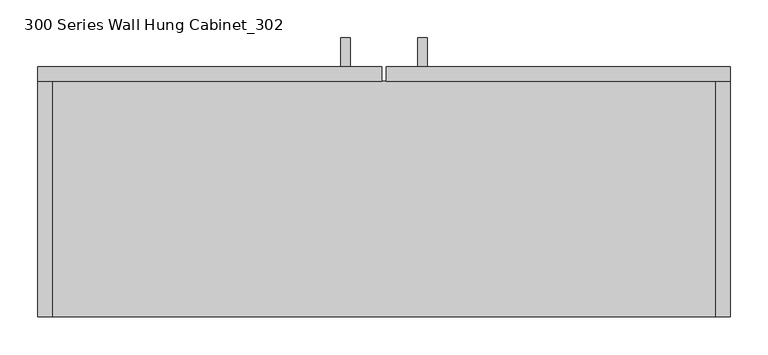
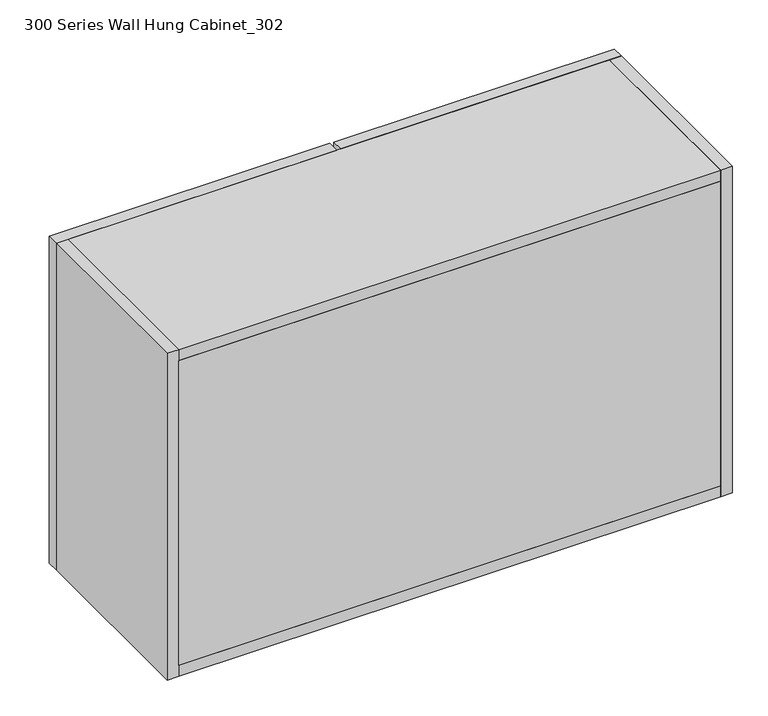
"""IFC4 building model written with IfcOpenShell, lengths in millimetres: furniture geometry, 300 Series Wall Hung Cabinet_302."""

import ifcopenshell
import ifcopenshell.guid

model = None  # the IFC model being written
_history = None  # IfcOwnerHistory: only IFC2X3 demands one
_inside = {}  # id of a spatial element -> (the spatial element, [elements in it])
_under = {}  # id of a project, library or spatial element -> (it, [spatial elements below it])
_declared = {}  # id of a project -> (the project, [libraries it declares])
_typed = {}  # id of a type object -> (the type object, [elements of that type])
_made_of = {}  # id of a material, layer set ... -> (it, [elements and type objects made of it])


def new_model(schema):
    """Start an empty IFC model of exactly this schema.

    Asked for "IFC4X3", IfcOpenShell would pick the latest addendum, in which some entities
    have other attributes; the version numbers below select the first issue.
    IFC2X3 requires an IfcOwnerHistory on every rooted entity: one is made here for all.
    """
    global model, _history
    if schema == "IFC4X3":
        model = ifcopenshell.file(schema_version=(4, 3, 0, 0))
    else:
        model = ifcopenshell.file(schema=schema)
    _inside.clear()
    _under.clear()
    _declared.clear()
    _typed.clear()
    _made_of.clear()
    _history = None
    if model.schema == "IFC2X3":
        org = make("IfcOrganization", Name="unknown")
        user = make(
            "IfcPersonAndOrganization",
            ThePerson=make("IfcPerson", FamilyName="unknown"),
            TheOrganization=org,
        )
        app = make(
            "IfcApplication",
            ApplicationDeveloper=org,
            Version="unknown",
            ApplicationFullName="unknown",
            ApplicationIdentifier="unknown",
        )
        _history = make(
            "IfcOwnerHistory",
            OwningUser=user,
            OwningApplication=app,
            ChangeAction="ADDED",
            CreationDate=0,
        )
    return model


def make(cls, **values):
    """One entity of the class cls with the attributes given. An attribute that is None is left unset."""
    return model.create_entity(
        cls, **{name: value for name, value in values.items() if value is not None}
    )


def rooted(cls, **values):
    """An entity with a GlobalId (a new one), such as an element, a storey or a relation."""
    return make(cls, GlobalId=ifcopenshell.guid.new(), OwnerHistory=_history, **values)


def si_unit(unit_type, name, prefix=None):
    """IfcSIUnit, for example si_unit("LENGTHUNIT", "METRE", prefix="MILLI")."""
    return make("IfcSIUnit", UnitType=unit_type, Prefix=prefix, Name=name)


def assignment(units):
    """IfcUnitAssignment: the units of a project."""
    return None if units is None else make("IfcUnitAssignment", Units=units)


def point(xyz):
    """IfcCartesianPoint."""
    return None if xyz is None else make("IfcCartesianPoint", Coordinates=xyz)


def direction(xyz):
    """IfcDirection."""
    return None if xyz is None else make("IfcDirection", DirectionRatios=xyz)


def frame(location, z_axis=None, x_axis=None):
    """IfcAxis2Placement3D, a coordinate frame: its origin and axes. An axis left out is left unset."""
    return make(
        "IfcAxis2Placement3D",
        Location=point(location),
        Axis=direction(z_axis),
        RefDirection=direction(x_axis),
    )


def origin():
    """The frame at (0, 0, 0) with its axes left unset."""
    return frame((0.0, 0.0, 0.0))


def place(relative_to, where):
    """IfcLocalPlacement: puts the frame where relative to a parent placement (None: the world)."""
    return make(
        "IfcLocalPlacement", PlacementRelTo=relative_to, RelativePlacement=where
    )


def context(
    kind, dimensions, precision=None, world=None, true_north=None, identifier=None
):
    """IfcGeometricRepresentationContext, for example the 3D "Model" context."""
    return make(
        "IfcGeometricRepresentationContext",
        ContextIdentifier=identifier,
        ContextType=kind,
        CoordinateSpaceDimension=dimensions,
        Precision=precision,
        WorldCoordinateSystem=world,
        TrueNorth=true_north,
    )


def project(units=None, contexts=None):
    """IfcProject with its units and contexts."""
    return rooted(
        "IfcProject",
        Name="project",
        RepresentationContexts=contexts,
        UnitsInContext=assignment(units),
    )


def spatial(cls, under=None, at=None, **own):
    """A site, building, storey or space (cls), placed at a placement, below another one or the project."""
    s = rooted(cls, ObjectPlacement=at, **own)
    if under is not None:
        _under.setdefault(under.id(), (under, []))[1].append(s)
    return s


def polyline(points):
    """IfcPolyline through the points."""
    return make("IfcPolyline", Points=[point(p) for p in points])


def outline(outer, holes=None, kind="AREA"):
    """IfcArbitraryClosedProfileDef: a profile drawn as a closed curve; with holes, ...WithVoids."""
    if holes is None:
        return make("IfcArbitraryClosedProfileDef", ProfileType=kind, OuterCurve=outer)
    return make(
        "IfcArbitraryProfileDefWithVoids",
        ProfileType=kind,
        OuterCurve=outer,
        InnerCurves=holes,
    )


def extrude(swept, where, along, depth):
    """IfcExtrudedAreaSolid: the profile swept, set in the frame where, extruded along a direction by depth."""
    return make(
        "IfcExtrudedAreaSolid",
        SweptArea=swept,
        Position=where,
        ExtrudedDirection=direction(along),
        Depth=depth,
    )


def shape(context_of_items, identifier, shape_type, items):
    """IfcShapeRepresentation: the items that make up one representation, for example the "Body"."""
    return make(
        "IfcShapeRepresentation",
        ContextOfItems=context_of_items,
        RepresentationIdentifier=identifier,
        RepresentationType=shape_type,
        Items=items,
    )


def source(mapping_origin, context_of_items, identifier, shape_type, items):
    """IfcRepresentationMap: a shape defined once, which mapped items show again and again."""
    return make(
        "IfcRepresentationMap",
        MappingOrigin=mapping_origin,
        MappedRepresentation=shape(context_of_items, identifier, shape_type, items),
    )


def transform(
    local_origin,
    x_axis=None,
    y_axis=None,
    z_axis=None,
    scale=None,
    scale2=None,
    scale3=None,
    uniform=True,
):
    """IfcCartesianTransformationOperator3D, or its non-uniform kind. x_axis, y_axis, z_axis: its Axis1, 2, 3."""
    if uniform:
        return make(
            "IfcCartesianTransformationOperator3D",
            Axis1=direction(x_axis),
            Axis2=direction(y_axis),
            LocalOrigin=point(local_origin),
            Scale=scale,
            Axis3=direction(z_axis),
        )
    return make(
        "IfcCartesianTransformationOperator3DnonUniform",
        Axis1=direction(x_axis),
        Axis2=direction(y_axis),
        LocalOrigin=point(local_origin),
        Scale=scale,
        Axis3=direction(z_axis),
        Scale2=scale2,
        Scale3=scale3,
    )


def mapped(mapping_source, mapping_target):
    """IfcMappedItem: shows the shape of a source again, moved by a transform."""
    return make(
        "IfcMappedItem", MappingSource=mapping_source, MappingTarget=mapping_target
    )


def made_of(thing, what):
    """Note that an element or type object is made of a material, layer set ...; save() writes the relation."""
    if what is not None:
        _made_of.setdefault(what.id(), (what, []))[1].append(thing)
    return thing


def element(
    cls,
    number,
    at=None,
    inside=None,
    cuts=None,
    type_object=None,
    material=None,
    context=None,
    identifier="Body",
    shape_type=None,
    held_by="IfcProductDefinitionShape",
    body=None,
    shapes=None,
    **own,
):
    """One element of the class cls, such as IfcWall. Its Tag is "e" and its number.

    at: its placement. inside: the storey or other place that contains it. cuts: it is an
    opening in that element (IfcRelVoidsElement). A single representation is given by context,
    identifier, shape_type and body (its items); several are given by shapes. held_by: the class
    of the entity that holds the representations. save() writes the other relations.
    """
    e = rooted(cls, Tag="e%d" % number, ObjectPlacement=at, **own)
    if body is not None:
        shapes = [shape(context, identifier, shape_type, body)]
    if shapes is not None:
        e.Representation = make(held_by, Representations=shapes)
    if inside is not None:
        _inside.setdefault(inside.id(), (inside, []))[1].append(e)
    if cuts is not None:
        rooted(
            "IfcRelVoidsElement", RelatingBuildingElement=cuts, RelatedOpeningElement=e
        )
    if type_object is not None:
        _typed.setdefault(type_object.id(), (type_object, []))[1].append(e)
    return made_of(e, material)


def aggregate(whole, parts):
    """IfcRelAggregates: a whole, such as a stair, and the parts it consists of."""
    return rooted("IfcRelAggregates", RelatingObject=whole, RelatedObjects=parts)


def save(model, path):
    """Write the relations noted so far, then the file.

    IfcRelAggregates (storeys below a building ...), IfcRelContainedInSpatialStructure (elements
    in a storey), IfcRelDefinesByType, IfcRelAssociatesMaterial and IfcRelDeclares: one each for
    every whole, place, type object, material and project.
    """
    for whole, parts in _under.values():
        aggregate(whole, parts)
    for where, things in _inside.values():
        rooted(
            "IfcRelContainedInSpatialStructure",
            RelatedElements=things,
            RelatingStructure=where,
        )
    for kind, things in _typed.values():
        rooted("IfcRelDefinesByType", RelatedObjects=things, RelatingType=kind)
    for what, things in _made_of.values():
        rooted("IfcRelAssociatesMaterial", RelatedObjects=things, RelatingMaterial=what)
    for by, libraries in _declared.values():
        rooted("IfcRelDeclares", RelatingContext=by, RelatedDefinitions=libraries)
    model.write(path)


def furniture_300_series_wall_hung_cabinet_302_73f347b2(model_context):
    return source(origin(), model_context, "Body", "SweptSolid", [
        extrude(outline(polyline([(406.4, 1708.1425373), (406.4, 1720.8121874), (444.4810937, 1720.8121874), (444.4810937, 1625.6), (406.4, 1625.6), (406.4, 1638.2696501), (431.8114436, 1638.2696501), (431.8114436, 1708.1425373), (406.4, 1708.1425373)])), frame((-57.15, 0.0, 0.0), z_axis=(1.0, 0.0, 0.0), x_axis=(0.0, 1.0, 0.0)), (0.0, 0.0, 1.0), 12.4065288),
        extrude(outline(polyline([(406.4, 1708.1425373), (406.4, 1720.8121874), (444.4810937, 1720.8121874), (444.4810937, 1625.6), (406.4, 1625.6), (406.4, 1638.2696501), (431.8114436, 1638.2696501), (431.8114436, 1708.1425373), (406.4, 1708.1425373)])), frame((44.45, 0.0, 0.0), z_axis=(1.0, 0.0, 0.0), x_axis=(0.0, 1.0, 0.0)), (0.0, 0.0, 1.0), 12.4065288),
        extrude(outline(polyline([(438.15, 76.2), (-438.15, 76.2), (-438.15, 95.25), (438.15, 95.25), (438.15, 76.2)])), frame((0.0, 0.0, 1593.85), z_axis=(0.0, 0.0, 1.0), x_axis=(1.0, 0.0, 0.0)), (0.0, 0.0, 1.0), 520.7),
        extrude(outline(polyline([(-3.175, 387.35), (-457.2, 387.35), (-457.2, 406.4), (-3.175, 406.4), (-3.175, 387.35)])), frame((0.0, 0.0, 1574.8), z_axis=(0.0, 0.0, 1.0), x_axis=(1.0, 0.0, 0.0)), (0.0, 0.0, 1.0), 558.8),
        extrude(outline(polyline([(457.2, 387.35), (3.175, 387.35), (3.175, 406.4), (457.2, 406.4), (457.2, 387.35)])), frame((0.0, 0.0, 1574.8), z_axis=(0.0, 0.0, 1.0), x_axis=(1.0, 0.0, 0.0)), (0.0, 0.0, 1.0), 558.8),
        extrude(outline(polyline([(-457.2, 76.2), (-457.2, 387.35), (-438.15, 387.35), (-438.15, 76.2), (-457.2, 76.2)])), frame((0.0, 0.0, 1574.8), z_axis=(0.0, 0.0, 1.0), x_axis=(1.0, 0.0, 0.0)), (0.0, 0.0, 1.0), 558.8),
        extrude(outline(polyline([(438.15, 76.2), (438.15, 387.35), (457.2, 387.35), (457.2, 76.2), (438.15, 76.2)])), frame((0.0, 0.0, 1574.8), z_axis=(0.0, 0.0, 1.0), x_axis=(1.0, 0.0, 0.0)), (0.0, 0.0, 1.0), 558.8),
        extrude(outline(polyline([(438.15, 387.35), (438.15, 76.2), (-438.15, 76.2), (-438.15, 387.35), (438.15, 387.35)])), frame((0.0, 0.0, 2114.55), z_axis=(0.0, 0.0, 1.0), x_axis=(1.0, 0.0, 0.0)), (0.0, 0.0, 1.0), 19.05),
        extrude(outline(polyline([(438.15, 387.35), (438.15, 76.2), (-438.15, 76.2), (-438.15, 387.35), (438.15, 387.35)])), frame((0.0, 0.0, 1574.8), z_axis=(0.0, 0.0, 1.0), x_axis=(1.0, 0.0, 0.0)), (0.0, 0.0, 1.0), 19.05),
    ])


if __name__ == "__main__":
    model = new_model("IFC4")
    model_context = context("Model", 3, world=origin())
    ifc_project = project(units=[si_unit("LENGTHUNIT", "METRE", prefix="MILLI")], contexts=[model_context])
    site = spatial("IfcSite", under=ifc_project)
    building = spatial("IfcBuilding", under=site)
    placement = place(None, origin())
    furniture_300_series_wall_hung_cabinet_302_shape = furniture_300_series_wall_hung_cabinet_302_73f347b2(model_context)
    element("IfcFurniture", 1, ObjectType="300 Series Wall Hung Cabinet_302 : 36\"W x 21\"H", at=placement, inside=building, context=model_context, shape_type="MappedRepresentation", body=[
        mapped(furniture_300_series_wall_hung_cabinet_302_shape, transform((0.0, 0.0, 0.0), x_axis=(1.0, 0.0, 0.0), y_axis=(0.0, 1.0, 0.0), z_axis=(0.0, 0.0, 1.0))),
    ])
    save(model, "model.ifc")

# Revit data of these elements
# Type "300 Series Wall Hung Cabinet_302 : 36\"W x 21\"H"
#   URL = "www.wicnet.org/manual_sections.asp"
#   Model = "302"
#   Manufacturer = "Woodwork Institute"
#   Description = "Wall Hung Cabinet"
#   Content Creator URL = "www.AECcontent.com"
#   Content Creator = "AECcontent"
#   Assembly Code = "E2010200"
#   Width = 3' - 0"
#   Top of Cabinet = 7' - 0"
#   Height = 1' - 10"
#   Depth = 1' - 1"
#   Top Panel Material = Cabinet
#   Side Panel Material = Cabinet
#   Shelf Panel Material = Cabinet
#   Door Panel Material = Cabinet
# Element 1 (IfcFurniture, "300 Series Wall Hung Cabinet_302 : 36\"W x 21\"H")
#   Materials on its faces: "Cabinet", "Default metal"
# Materials
#   "Cabinet": class "Wood", colour RGB 189 170 130, transparency 0, Cost = 0
#   "Default metal": class "Unassigned", colour RGB 204 204 204, transparency 0
